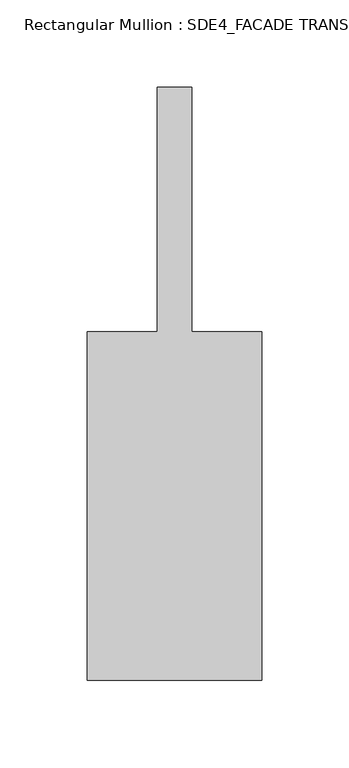
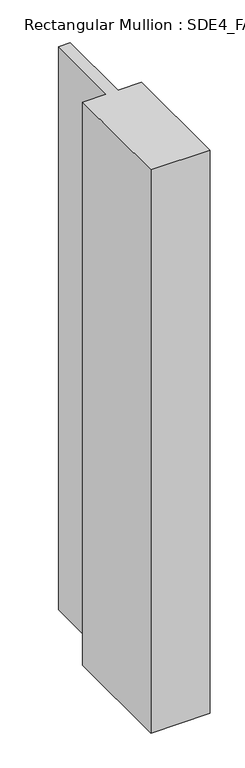
"""IFC4 building model written with IfcOpenShell, lengths in millimetres: member geometry, Rectangular Mullion : SDE4_FACADE TRANSOM TYPE 1."""

from ifc_helpers import new_model, si_unit, frame, origin, place, context, project, spatial, polyline, outline, extrude, source, transform, mapped, element, save


def rectangular_mullion_sde4_facade_transom_type_1_eba76ebd(model_context):
    return source(origin(), model_context, "Body", "SweptSolid", [
        extrude(outline(polyline([(50.0, -132.5), (-50.0, -132.5), (-50.0, 67.5), (-10.0, 67.5), (-10.0, 207.5), (10.0, 207.5), (10.0, 67.5), (50.0, 67.5), (50.0, -132.5)])), frame((0.0, 0.0, -1005.6182871), z_axis=(0.0, 0.0, 1.0), x_axis=(1.0, 0.0, 0.0)), (0.0, 0.0, 1.0), 1005.6182871),
    ])


if __name__ == "__main__":
    model = new_model("IFC4")
    model_context = context("Model", 3, world=origin())
    ifc_project = project(units=[si_unit("LENGTHUNIT", "METRE", prefix="MILLI")], contexts=[model_context])
    site = spatial("IfcSite", under=ifc_project)
    building = spatial("IfcBuilding", under=site)
    placement = place(None, origin())
    rectangular_mullion_sde4_facade_transom_type_1_shape = rectangular_mullion_sde4_facade_transom_type_1_eba76ebd(model_context)
    element("IfcMember", 1, ObjectType="Rectangular Mullion : SDE4_FACADE TRANSOM TYPE 1", at=placement, inside=building, context=model_context, shape_type="MappedRepresentation", body=[
        mapped(rectangular_mullion_sde4_facade_transom_type_1_shape, transform((0.0, 0.0, 0.0), x_axis=(1.0, 0.0, 0.0), y_axis=(0.0, 1.0, 0.0), z_axis=(0.0, 0.0, 1.0))),
    ])
    save(model, "model.ifc")

# Revit data of these elements
# Type "Rectangular Mullion : SDE4_FACADE TRANSOM TYPE 1"
#   built-in parameter 1007322 = 1.11549 (stored number, unit not read)
#   built-in parameter 1007321 = 0.164042 (stored number, unit not read)
#   built-in parameter 1007320 = 0.164042 (stored number, unit not read)
